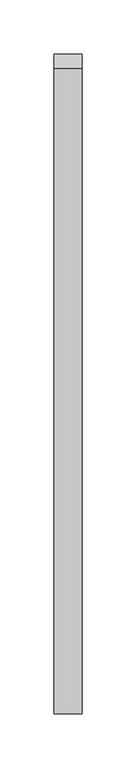
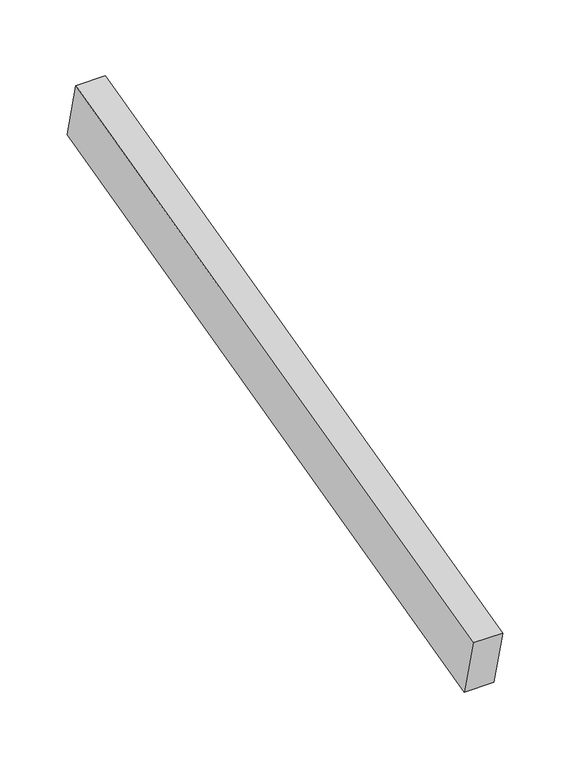
"""IFC4 building model written with IfcOpenShell, lengths in millimetres: proxy geometry, Roof006 1035 : Roof006 1035."""

from ifc_helpers import new_model, si_unit, frame, origin, place, context, project, spatial, polyline, outline, extrude, source, transform, mapped, element, save


def generic_models_7305a674(model_context):
    return source(origin(), model_context, "Body", "SweptSolid", [
        extrude(outline(polyline([(10169.6304502, 43758.3868694), (10156.4176865, 43811.2379242), (10748.8728775, 43959.34982), (10762.0851937, 43906.5005553), (10169.6304502, 43758.3868694)])), frame((5168.9879286, 0.0, 0.0), z_axis=(1.0, 0.0, 0.0), x_axis=(0.0, 1.0, 0.0)), (0.0, 0.0, 1.0), 25.4),
    ])


if __name__ == "__main__":
    model = new_model("IFC4")
    model_context = context("Model", 3, world=origin())
    ifc_project = project(units=[si_unit("LENGTHUNIT", "METRE", prefix="MILLI")], contexts=[model_context])
    site = spatial("IfcSite", under=ifc_project)
    building = spatial("IfcBuilding", under=site)
    placement = place(None, origin())
    generic_models_shape = generic_models_7305a674(model_context)
    element("IfcBuildingElementProxy", 1, Name="Roof006 1035 : Roof006 1035", ObjectType="Roof006 1035 : Roof006 1035", at=placement, inside=building, context=model_context, shape_type="MappedRepresentation", body=[
        mapped(generic_models_shape, transform((0.0, 0.0, 0.0), x_axis=(1.0, 0.0, 0.0), y_axis=(0.0, 1.0, 0.0), z_axis=(0.0, 0.0, 1.0))),
    ])
    save(model, "model.ifc")

# Revit data of these elements
# Type "Roof006 1035 : Roof006 1035"
#   NameOverride = "Roof006"
# Element 1 (IfcBuildingElementProxy, "Roof006 1035 : Roof006 1035")
#   Materials on its faces: "STANDING SEAM METAL ROOF"
# Materials
#   "STANDING SEAM METAL ROOF": class "Unassigned", colour RGB 128 128 128, transparency 0
